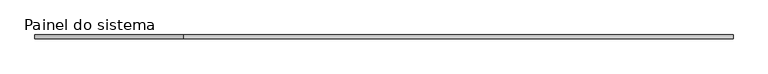
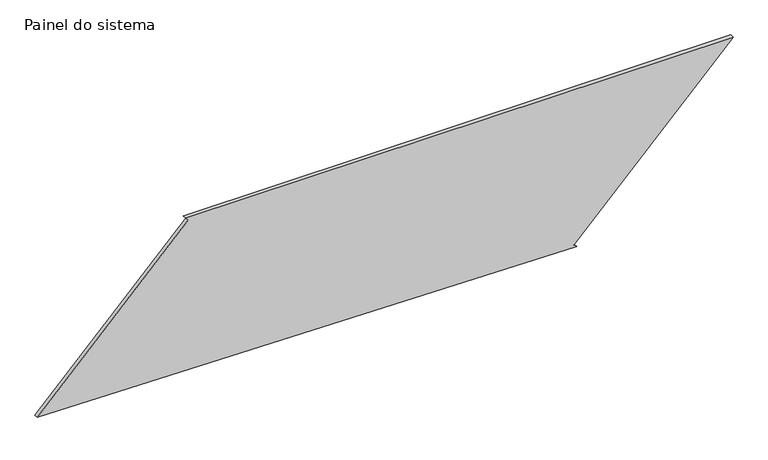
"""IFC4 building model written with IfcOpenShell, lengths in millimetres: plate geometry, Painel do sistema : Envidraçado."""

from ifc_helpers import new_model, si_unit, frame, origin, place, context, project, spatial, polyline, outline, extrude, source, transform, mapped, element, save


def painel_do_sistema_1aaf07c6(model_context):
    return source(origin(), model_context, "Body", "SweptSolid", [
        extrude(outline(polyline([(0.0, 1241.1732003), (17.3932625, 1223.2156276), (1081.9766835, 2254.3449029), (1081.9766835, -1292.3885253), (1064.5834209, -1274.4309526), (52.8769643, -2254.3449029), (0.0, 1241.1732003)])), frame((0.0, 24.5, 0.0), z_axis=(0.0, 1.0, 0.0), x_axis=(0.0, 0.0, 1.0)), (0.0, 0.0, 1.0), 25.0),
    ])


if __name__ == "__main__":
    model = new_model("IFC4")
    model_context = context("Model", 3, world=origin())
    ifc_project = project(units=[si_unit("LENGTHUNIT", "METRE", prefix="MILLI")], contexts=[model_context])
    site = spatial("IfcSite", under=ifc_project)
    building = spatial("IfcBuilding", under=site)
    placement = place(None, origin())
    painel_do_sistema_shape = painel_do_sistema_1aaf07c6(model_context)
    element("IfcPlate", 1, ObjectType="Painel do sistema : Envidraçado", at=placement, inside=building, context=model_context, shape_type="MappedRepresentation", body=[
        mapped(painel_do_sistema_shape, transform((0.0, 0.0, 0.0), x_axis=(1.0, 0.0, 0.0), y_axis=(0.0, 1.0, 0.0), z_axis=(0.0, 0.0, 1.0))),
    ])
    save(model, "model.ifc")

# Revit data of these elements
# Type "Painel do sistema : Envidraçado"
#   Construction Type Id = "GSP4R"
#   Analytic Construction = "Vidraça única Pilkington 1/8 pol"
#   Visual Light Transmittance = 0.9
#   Solar Heat Gain Coefficient = 0.86
#   Heat Transfer Coefficient (U) = 6.7069 W/(m²·K)
# Element 1 (IfcPlate, "Painel do sistema : Envidraçado")
#   Materials on its faces: "Vidro"
# Materials
#   "Vidro": class "Vidro", colour RGB 0 128 192, transparency 0.9, Description = "Vidro de sílica", Cost = 0
